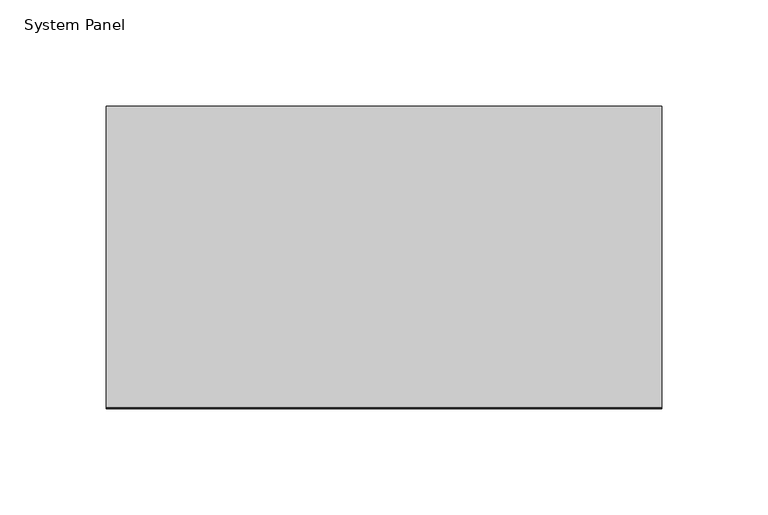
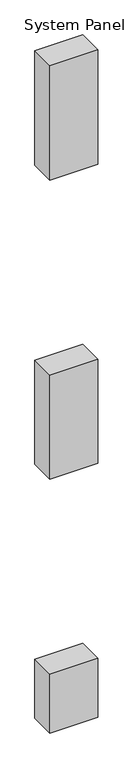
"""IFC4 building model written with IfcOpenShell, lengths in millimetres: plate geometry, System Panel : NLRS_21_CWP_hsb-vulling minerale wol 142 _gen_rsf."""

from ifc_helpers import new_model, si_unit, frame, origin, origin_with_axes, place, context, project, spatial, polyline, outline, extrude, source, transform, mapped, element, save


def system_panel_51be6294(model_context):
    return source(origin(), model_context, "Body", "SweptSolid", [
        extrude(outline(polyline([(131.0, -71.0), (-131.0, -71.0), (-131.0, 71.0), (131.0, 71.0), (131.0, -71.0)])), origin_with_axes(), (0.0, 0.0, 1.0), 339.0),
        extrude(outline(polyline([(131.0, -71.0), (-131.0, -71.0), (-131.0, 71.0), (131.0, 71.0), (131.0, -71.0)])), frame((0.0, 0.0, 1465.0), z_axis=(0.0, 0.0, 1.0), x_axis=(1.0, 0.0, 0.0)), (0.0, 0.0, 1.0), 599.0),
        extrude(outline(polyline([(131.0, -71.0), (-131.0, -71.0), (-131.0, 71.0), (131.0, 71.0), (131.0, -71.0)])), frame((0.0, 0.0, 3190.0), z_axis=(0.0, 0.0, 1.0), x_axis=(1.0, 0.0, 0.0)), (0.0, 0.0, 1.0), 659.0),
    ])


if __name__ == "__main__":
    model = new_model("IFC4")
    model_context = context("Model", 3, world=origin())
    ifc_project = project(units=[si_unit("LENGTHUNIT", "METRE", prefix="MILLI")], contexts=[model_context])
    site = spatial("IfcSite", under=ifc_project)
    building = spatial("IfcBuilding", under=site)
    placement = place(None, origin())
    system_panel_shape = system_panel_51be6294(model_context)
    element("IfcPlate", 1, ObjectType="System Panel : NLRS_21_CWP_hsb-vulling minerale wol 142 _gen_rsf", at=placement, inside=building, context=model_context, shape_type="MappedRepresentation", body=[
        mapped(system_panel_shape, transform((0.0, 0.0, 0.0), x_axis=(1.0, 0.0, 0.0), y_axis=(0.0, 1.0, 0.0), z_axis=(0.0, 0.0, 1.0))),
    ])
    save(model, "model.ifc")

# Revit data of these elements
# Type "System Panel : NLRS_21_CWP_hsb-vulling minerale wol 142 _gen_rsf"
#   Export Type to IFC As = "IfcWall"
#   Type IfcGUID = "07M7mRoiH1CR8m_RSKIwpC"
#   Assembly Code = "21.23"
# Element 1 (IfcPlate, "System Panel : NLRS_21_CWP_hsb-vulling minerale wol 142 _gen_rsf")
#   Materials on its faces: "NLRS_m1_isolatie minerale wol_gen_rsf"
# Materials
#   "NLRS_m1_isolatie minerale wol_gen_rsf": class "M - Anorganische materialen", colour RGB 200 200 140, transparency 0, Keynote = "m1", Manufacturer = "Revit Standards Foundation", URL = "www.revitstandards.org", Description = "isolatie minerale wol", Cost = 0
